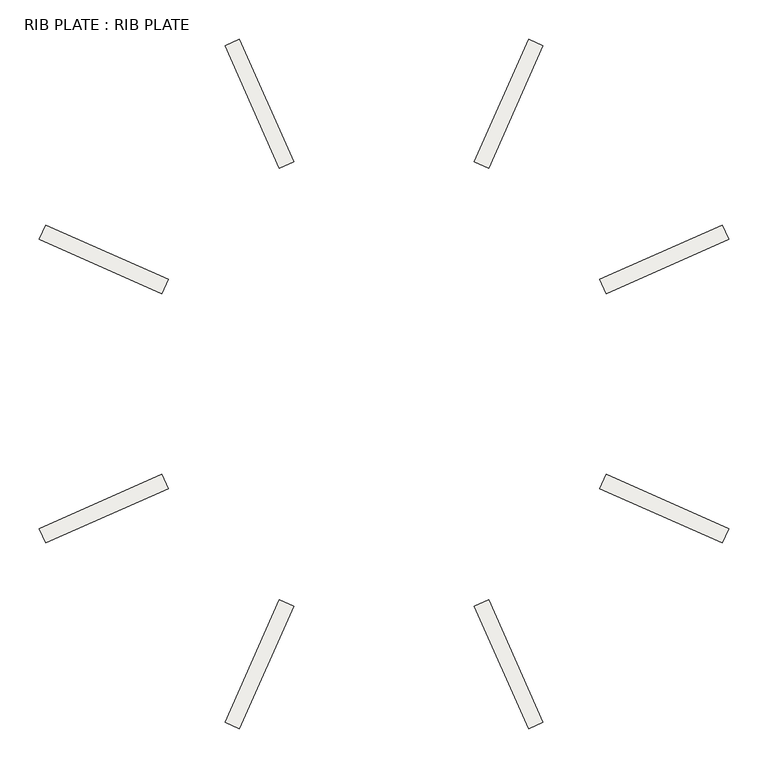
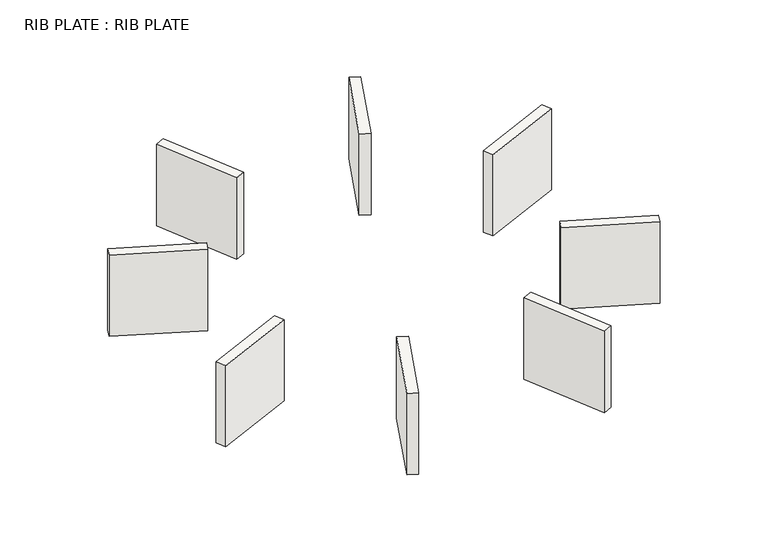
"""IFC4 building model written with IfcOpenShell, lengths in millimetres: slab geometry, RIB PLATE : RIB PLATE."""

from ifc_helpers import new_model, si_unit, frame, origin, place, context, project, spatial, polyline, outline, extrude, source, transform, mapped, element, save


def rib_plate_rib_plate_03f79d07(model_context):
    return source(origin(), model_context, "Body", "SweptSolid", [
        extrude(outline(polyline([(-183.5745867, 19937.1858234), (-114.5310474, 19781.8378601), (-132.8072784, 19773.7150908), (-201.8508176, 19929.063054), (-183.5745867, 19937.1858234)])), frame((0.0, 0.0, 40.0002155), z_axis=(0.0, 0.0, 1.0), x_axis=(1.0, 0.0, 0.0)), (0.0, 0.0, 1.0), 170.0),
        extrude(outline(polyline([(429.5421952, 19297.6700413), (274.1942319, 19366.7135805), (282.3170012, 19384.9898115), (437.6649645, 19315.9462722), (429.5421952, 19297.6700413)])), frame((0.0, 0.0, 40.0002155), z_axis=(0.0, 0.0, 1.0), x_axis=(1.0, 0.0, 0.0)), (0.0, 0.0, 1.0), 170.0),
        extrude(outline(polyline([(437.6649645, 19683.0954455), (282.3170012, 19614.0519063), (274.1942319, 19632.3281373), (429.5421952, 19701.3716765), (437.6649645, 19683.0954455)])), frame((0.0, 0.0, 40.0002155), z_axis=(0.0, 0.0, 1.0), x_axis=(1.0, 0.0, 0.0)), (0.0, 0.0, 1.0), 170.0),
        extrude(outline(polyline([(201.8508176, 19929.063054), (132.8072784, 19773.7150908), (114.5310474, 19781.8378601), (183.5745867, 19937.1858234), (201.8508176, 19929.063054)])), frame((0.0, 0.0, 40.0002155), z_axis=(0.0, 0.0, 1.0), x_axis=(1.0, 0.0, 0.0)), (0.0, 0.0, 1.0), 170.0),
        extrude(outline(polyline([(-429.5421952, 19701.3716765), (-274.1942319, 19632.3281373), (-282.3170012, 19614.0519063), (-437.6649645, 19683.0954455), (-429.5421952, 19701.3716765)])), frame((0.0, 0.0, 40.0002155), z_axis=(0.0, 0.0, 1.0), x_axis=(1.0, 0.0, 0.0)), (0.0, 0.0, 1.0), 170.0),
        extrude(outline(polyline([(-437.6649645, 19315.9462722), (-282.3170012, 19384.9898115), (-274.1942319, 19366.7135805), (-429.5421952, 19297.6700413), (-437.6649645, 19315.9462722)])), frame((0.0, 0.0, 40.0002155), z_axis=(0.0, 0.0, 1.0), x_axis=(1.0, 0.0, 0.0)), (0.0, 0.0, 1.0), 170.0),
        extrude(outline(polyline([(-201.8508176, 19069.9786637), (-132.8072784, 19225.326627), (-114.5310474, 19217.2038577), (-183.5745867, 19061.8558944), (-201.8508176, 19069.9786637)])), frame((0.0, 0.0, 40.0002155), z_axis=(0.0, 0.0, 1.0), x_axis=(1.0, 0.0, 0.0)), (0.0, 0.0, 1.0), 170.0),
        extrude(outline(polyline([(183.5745867, 19061.8558944), (114.5310474, 19217.2038577), (132.8072784, 19225.326627), (201.8508176, 19069.9786637), (183.5745867, 19061.8558944)])), frame((0.0, 0.0, 40.0002155), z_axis=(0.0, 0.0, 1.0), x_axis=(1.0, 0.0, 0.0)), (0.0, 0.0, 1.0), 170.0),
    ])


if __name__ == "__main__":
    model = new_model("IFC4")
    model_context = context("Model", 3, world=origin())
    ifc_project = project(units=[si_unit("LENGTHUNIT", "METRE", prefix="MILLI")], contexts=[model_context])
    site = spatial("IfcSite", under=ifc_project)
    building = spatial("IfcBuilding", under=site)
    placement = place(None, origin())
    rib_plate_rib_plate_shape = rib_plate_rib_plate_03f79d07(model_context)
    element("IfcSlab", 1, ObjectType="RIB PLATE : RIB PLATE", at=placement, inside=building, context=model_context, shape_type="MappedRepresentation", body=[
        mapped(rib_plate_rib_plate_shape, transform((0.0, 0.0, 0.0), x_axis=(1.0, 0.0, 0.0), y_axis=(0.0, 1.0, 0.0), z_axis=(0.0, 0.0, 1.0))),
    ])
    save(model, "model.ifc")
